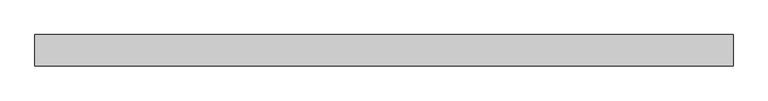
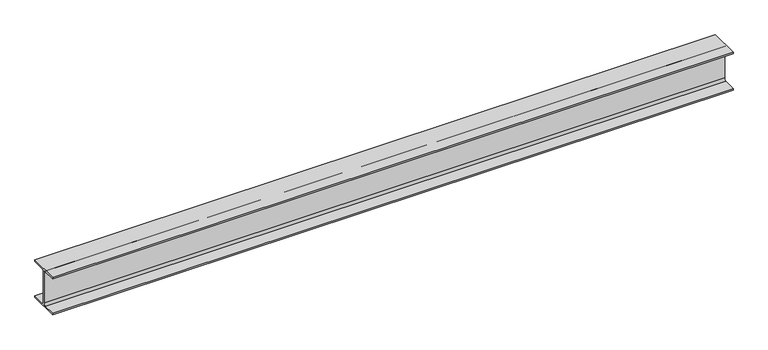
"""IFC4 building model written with IfcOpenShell, lengths in millimetres: beam geometry, 0912_Steel Framing_H-KSD3502 : H_SB_ASB_H-390x300x10x16."""

from ifc_helpers import new_model, si_unit, point, frame, frame_2d, origin, place, context, project, spatial, polyline, circle_curve, trimmed, segment, composite_curve, outline, extrude, source, transform, mapped, element, save


def beam_02203127(model_context):
    return source(origin(), model_context, "Body", "SweptSolid", [
        extrude(outline(composite_curve([segment(polyline([(150.0, -179.0), (150.0, -195.0), (-150.0, -195.0), (-150.0, -179.0), (-27.0, -179.0)]), True, "CONTINUOUS"), segment(trimmed(circle_curve(frame_2d((-27.0, -157.0)), 22.0), [point((-27.0, -179.0))], [point((-5.0, -157.0))], True, "CARTESIAN"), True, "CONTINUOUS"), segment(polyline([(-5.0, -157.0), (-5.0, 157.0)]), True, "CONTINUOUS"), segment(trimmed(circle_curve(frame_2d((-27.0, 157.0)), 22.0), [point((-5.0, 157.0))], [point((-27.0, 179.0))], True, "CARTESIAN"), True, "CONTINUOUS"), segment(polyline([(-27.0, 179.0), (-150.0, 179.0), (-150.0, 195.0), (150.0, 195.0), (150.0, 179.0), (27.0, 179.0)]), True, "CONTINUOUS"), segment(trimmed(circle_curve(frame_2d((27.0, 157.0)), 22.0), [point((27.0, 179.0))], [point((5.0, 157.0))], True, "CARTESIAN"), True, "CONTINUOUS"), segment(polyline([(5.0, 157.0), (5.0, -157.0)]), True, "CONTINUOUS"), segment(trimmed(circle_curve(frame_2d((27.0, -157.0)), 22.0), [point((5.0, -157.0))], [point((27.0, -179.0))], True, "CARTESIAN"), True, "CONTINUOUS"), segment(polyline([(27.0, -179.0), (150.0, -179.0)]), True, "CONTINUOUS")], self_intersect=False)), frame((-3337.3, 0.0, 0.0), z_axis=(1.0, 0.0, 0.0), x_axis=(0.0, 1.0, 0.0)), (0.0, 0.0, 1.0), 6674.6),
    ])


if __name__ == "__main__":
    model = new_model("IFC4")
    model_context = context("Model", 3, world=origin())
    ifc_project = project(units=[si_unit("LENGTHUNIT", "METRE", prefix="MILLI")], contexts=[model_context])
    site = spatial("IfcSite", under=ifc_project)
    building = spatial("IfcBuilding", under=site)
    placement = place(None, origin())
    beam_shape = beam_02203127(model_context)
    element("IfcBeam", 1, ObjectType="0912_Steel Framing_H-KSD3502 : H_SB_ASB_H-390x300x10x16", at=placement, inside=building, context=model_context, shape_type="MappedRepresentation", body=[
        mapped(beam_shape, transform((0.0, 0.0, 0.0), x_axis=(1.0, 0.0, 0.0), y_axis=(0.0, 1.0, 0.0), z_axis=(0.0, 0.0, 1.0))),
    ])
    save(model, "model.ifc")

# Revit data of these elements
# Type "0912_Steel Framing_H-KSD3502 : H_SB_ASB_H-390x300x10x16"
#   H_WM Code_1 = "S01AA001-00001 | Main Steel Structure Fabrication Work | Shelter/Building | Heavy Steel - Standard (Weight≥90KG/M) | Material: (   )"
#   H_WM Code_2 = "S03AA027-00001 | Main Steel Structure Erection Work | Shelter/Building | Heavy Steel (Weight≥90KG/M) | Material: (   )"
#   H_WM Code_3 = "S01AA010-00001 | Main Steel Structure Fabrication Work | Shelter/Building | Steel Painting/Coating | for Non-Fireproofed Steel Surface, Surface Preparation, Primer, Second & Final Coat | Material: (   )"
#   H_Q'ty Cal Type Tag = "SB-Q2"
#   Width = 30.0 cm
#   Web Thickness = 1.0 cm
#   Web Fillet = 2.2 cm
#   Warping Constant = 2520000.0 cm⁶
#   W = 0
#   Torsional Moment of Inertia = 94.3867 cm⁴
#   Section Area = 136.0 cm²
#   Plastic Modulus weak axis = 733.0 cm³
#   Plastic Modulus strong axis = 2190.0 cm³
#   Perimeter = 1.92 m²/m
#   Nominal Weight = 107.00 kgf/m
#   Moment of Inertia weak axis = 7210.00 cm⁴
#   Moment of Inertia strong axis = 38700.00 cm⁴
#   Height = 39.0 cm
#   Flange Thickness = 1.6 cm
#   Elastic Modulus weak axis = 481.0 cm³
#   Elastic Modulus strong axis = 1980.0 cm³
#   Centroid Vertical = 19.5 cm
#   Centroid Horizontal = 15.0 cm
#   Ix = 387000000
#   Length [instance default] = 1.5240 m
#   Zx = 2190000
#   b = 0.3000 m
#   h = 0.3900 m
#   r = 0.0220 m
#   s = 0.0100 m
#   t = 0.0160 m
#   A = 0.0136 m²
#   Structural Material [instance default] = Steel, 45-345
#   Assembly Code = ""
# Element 1 (IfcBeam, "0912_Steel Framing_H-KSD3502 : H_SB_ASB_H-390x300x10x16")
#   Structural Material = none
# Materials
#   "Steel, 45-345": class "Metal", colour RGB 189 187 185, transparency 0, Description = "Steel 345 MPa", Cost = 0
